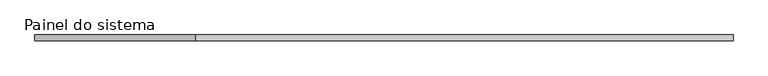
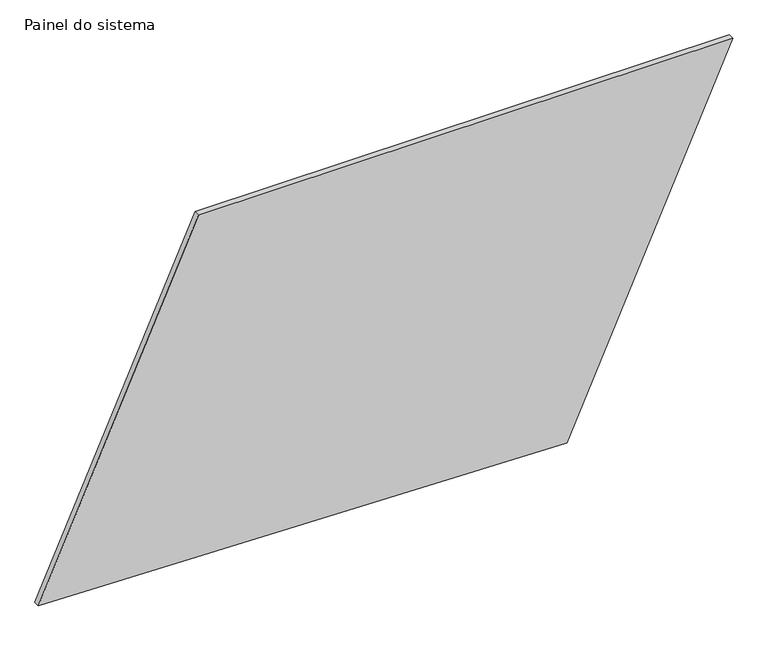
"""IFC4 building model written with IfcOpenShell, lengths in millimetres: plate geometry, Painel do sistema : Envidraçado."""

from ifc_helpers import new_model, si_unit, frame, origin, place, context, project, spatial, polyline, outline, extrude, source, transform, mapped, element, save


def painel_do_sistema_9cdced0e(model_context):
    return source(origin(), model_context, "Body", "SweptSolid", [
        extrude(outline(polyline([(54.3610064, -1468.6062494), (0.0, 766.7189198), (1565.0871093, 1468.6062494), (1565.0871093, -791.0979473), (54.3610064, -1468.6062494)])), frame((0.0, 24.5, 0.0), z_axis=(0.0, 1.0, 0.0), x_axis=(0.0, 0.0, 1.0)), (0.0, 0.0, 1.0), 25.0),
    ])


if __name__ == "__main__":
    model = new_model("IFC4")
    model_context = context("Model", 3, world=origin())
    ifc_project = project(units=[si_unit("LENGTHUNIT", "METRE", prefix="MILLI")], contexts=[model_context])
    site = spatial("IfcSite", under=ifc_project)
    building = spatial("IfcBuilding", under=site)
    placement = place(None, origin())
    painel_do_sistema_shape = painel_do_sistema_9cdced0e(model_context)
    element("IfcPlate", 1, ObjectType="Painel do sistema : Envidraçado", at=placement, inside=building, context=model_context, shape_type="MappedRepresentation", body=[
        mapped(painel_do_sistema_shape, transform((0.0, 0.0, 0.0), x_axis=(1.0, 0.0, 0.0), y_axis=(0.0, 1.0, 0.0), z_axis=(0.0, 0.0, 1.0))),
    ])
    save(model, "model.ifc")

# Revit data of these elements
# Type "Painel do sistema : Envidraçado"
#   Construction Type Id = "GSP4R"
#   Analytic Construction = "Vidraça única Pilkington 1/8 pol"
#   Visual Light Transmittance = 0.9
#   Solar Heat Gain Coefficient = 0.86
#   Heat Transfer Coefficient (U) = 6.7069 W/(m²·K)
# Element 1 (IfcPlate, "Painel do sistema : Envidraçado")
#   Materials on its faces: "Vidro"
# Materials
#   "Vidro": class "Vidro", colour RGB 0 128 192, transparency 0.9, Description = "Vidro de sílica", Cost = 0
